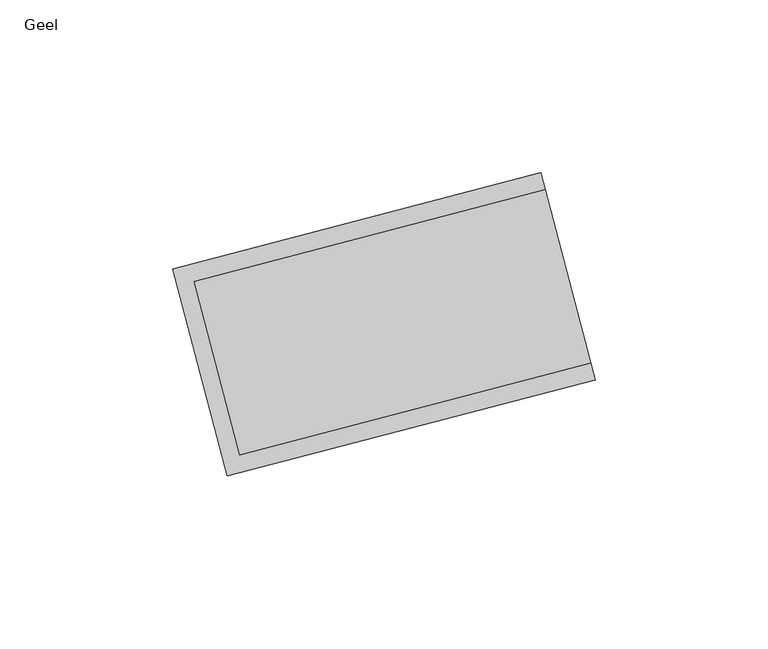
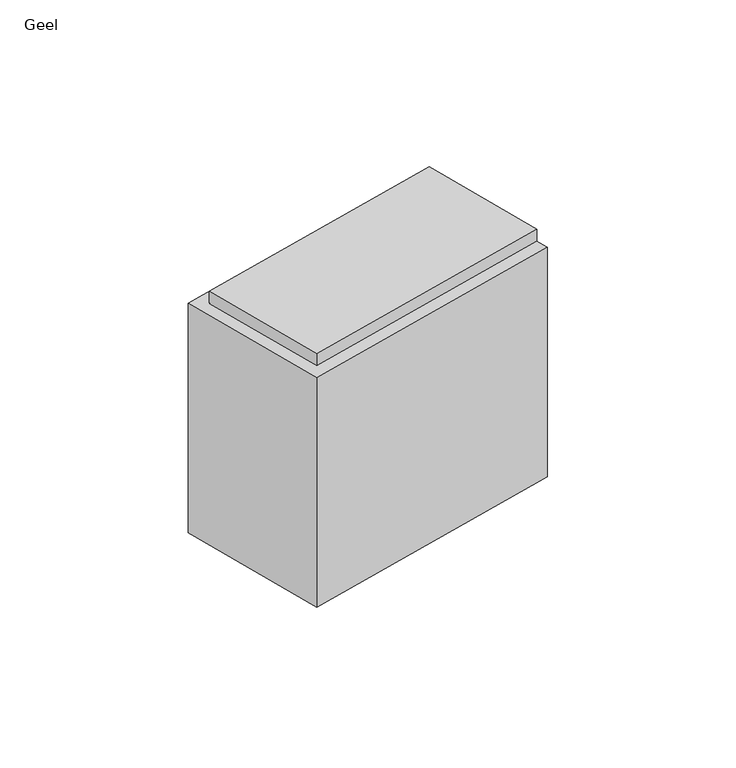
"""IFC4 building model written with IfcOpenShell, lengths in millimetres: proxy geometry, 00_GMA_steen_versie_6 : Geel."""

from ifc_helpers import new_model, si_unit, origin, origin_with_axes, place, context, project, spatial, polyline, outline, extrude, source, transform, mapped, element, save


def geel_ff5a4212(model_context):
    return source(origin(), model_context, "Body", "SweptSolid", [
        extrude(outline(polyline([(24.8461542, 24.0369432), (9.1731432, 83.919349), (115.5141152, 111.7519519), (116.7801202, 106.9148835), (15.2762167, 80.3482856), (28.4172176, 30.1400167), (129.9211211, 56.7066146), (131.1871262, 51.8695461), (24.8461542, 24.0369432)])), origin_with_axes(), (0.0, 0.0, 1.0), 95.0),
        extrude(outline(polyline([(116.7801202, 106.9148835), (129.9211211, 56.7066146), (28.4172176, 30.1400167), (15.2762167, 80.3482856), (116.7801202, 106.9148835)])), origin_with_axes(), (0.0, 0.0, 1.0), 100.0),
    ])


if __name__ == "__main__":
    model = new_model("IFC4")
    model_context = context("Model", 3, world=origin())
    ifc_project = project(units=[si_unit("LENGTHUNIT", "METRE", prefix="MILLI")], contexts=[model_context])
    site = spatial("IfcSite", under=ifc_project)
    building = spatial("IfcBuilding", under=site)
    placement = place(None, origin())
    geel_shape = geel_ff5a4212(model_context)
    element("IfcBuildingElementProxy", 1, Name="00_GMA_steen_versie_6 : Geel", ObjectType="00_GMA_steen_versie_6 : Geel", at=placement, inside=building, context=model_context, shape_type="MappedRepresentation", body=[
        mapped(geel_shape, transform((0.0, 0.0, 0.0), x_axis=(1.0, 0.0, 0.0), y_axis=(0.0, 1.0, 0.0), z_axis=(0.0, 0.0, 1.0))),
    ])
    save(model, "model.ifc")

# Revit data of these elements
# Type "00_GMA_steen_versie_6 : Geel"
#   Voegdikte = 95 mm
#   VoegTovSteen = -5 mm
#   StootvoegLinksHalfOnder [instance default] = 5 mm
#   StootvoegLinksHalfBoven [instance default] = 5 mm
#   StootVoegRechtsHalfOnder [instance default] = 5 mm
#   StootVoegRechtsHalfBoven [instance default] = 5 mm
#   StootVoegBreedteRechts [instance default] = 10 mm
#   StootVoegBreedteLinks [instance default] = 10 mm
#   Steendikte = 100 mm
#   LintVoegOnderHalf [instance default] = 0 mm
#   LintVoegOnder [instance default] = 0 mm
#   LintVoegBovenHalf [instance default] = 5 mm
#   LintVoegBoven [instance default] = 10 mm
#   materiaal = 21_steen_geel
#   MateriaalVoeg = 20_voeg
#   Default Elevation = 0
# Element 1 (IfcBuildingElementProxy, "00_GMA_steen_versie_6 : Geel")
#   StootVoegRechtsHalfOnder = 0 mm
#   StootVoegRechtsHalfBoven = 0 mm
#   StootVoegBreedteRechts = 0 mm
#   LintVoegOnderHalf = 5 mm
#   LintVoegOnder = 10 mm
#   Materials on its faces: "20_voeg", "21_steen_geel"
# Materials
#   "21_steen_geel": class "Unassigned", colour RGB 202 202 0, transparency 0, Cost = 0
#   "20_voeg": class "Concrete", colour RGB 86 86 86, transparency 0, Manufacturer = "RevitGG", URL = "www.revitgg.nl", Description = "zandcement, generiek materiaal", Cost = 0
